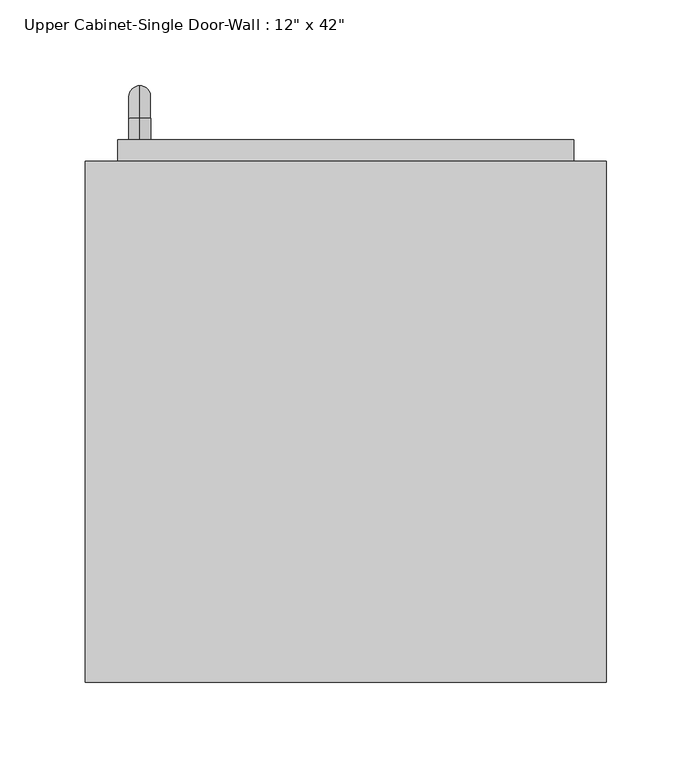
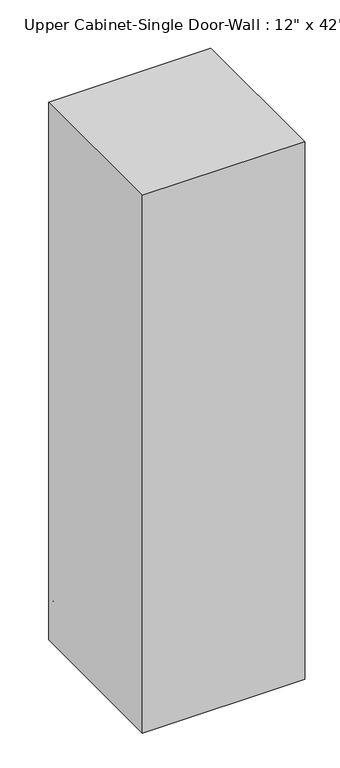
"""IFC4 building model written with IfcOpenShell, lengths in millimetres: furniture geometry."""

from ifc_helpers import new_model, si_unit, point, frame, origin, place, context, project, spatial, polyline, circle_curve, ellipse_curve, trimmed, outline, extrude, faceted_brep, source, transform, mapped, element, save
from ifc_brep_helpers import plane_surface, cylinder_surface, revolved_surface, advanced_brep


def furniture_d980f7c4(model_context):
    return source(origin(), model_context, "Body", "SolidModel", [
        faceted_brep([(-122.6288372, 61.9125, 2438.4), (-122.6288372, 61.9125, 1371.6), (182.1711628, 61.9125, 1371.6), (182.1711628, 61.9125, 2438.4), (-122.6288372, 366.7125, 2438.4), (182.1711628, 366.7125, 2438.4), (182.1711628, 366.7125, 1371.6), (-122.6288372, 366.7125, 1371.6), (-103.5788372, 366.7125, 2419.35), (-103.5788372, 366.7125, 1390.65), (163.1211628, 366.7125, 1390.65), (163.1211628, 366.7125, 2419.35), (163.1211628, 80.9625, 2419.35), (-103.5788372, 80.9625, 2419.35), (163.1211628, 80.9625, 1390.65), (-103.5788372, 80.9625, 1390.65)], [[[0, 1, 2, 3]], [[4, 5, 6, 7], [8, 9, 10, 11]], [[1, 0, 4, 7]], [[2, 1, 7, 6]], [[3, 2, 6, 5]], [[0, 3, 5, 4]], [[8, 11, 12, 13]], [[11, 10, 14, 12]], [[10, 9, 15, 14]], [[9, 8, 13, 15]], [[13, 12, 14, 15]]]),
        advanced_brep(
        [(-90.8788372, 379.4125, 1517.65), (-90.8788372, 379.4125, 1530.35), (-90.8788372, 392.1125, 1517.65), (-90.8788372, 392.1125, 1530.35), (-90.8788372, 411.1625, 1511.3), (-90.8788372, 398.4625, 1511.3), (-90.8788372, 398.4625, 1435.1), (-90.8788372, 411.1625, 1435.1), (-90.8788372, 392.1125, 1416.05), (-90.8788372, 392.1125, 1428.75), (-90.8788372, 379.4125, 1428.75), (-90.8788372, 379.4125, 1416.05)],
        [
            (0, 1, circle_curve(frame((-90.8788372, 379.4125, 1524.0), z_axis=(0.0, -1.0, 0.0), x_axis=(0.0, 0.0, 1.0)), 6.35)),
            (1, 0, circle_curve(frame((-90.8788372, 379.4125, 1524.0), z_axis=(0.0, -1.0, 0.0), x_axis=(0.0, 0.0, 1.0)), 6.35)),
            (0, 2),
            (2, 3, circle_curve(frame((-90.8788372, 392.1125, 1524.0), z_axis=(0.0, -1.0, 0.0), x_axis=(0.0, 0.0, 1.0)), 6.35)),
            (3, 1),
            (3, 2, circle_curve(frame((-90.8788372, 392.1125, 1524.0), z_axis=(0.0, -1.0, 0.0), x_axis=(0.0, 0.0, 1.0)), 6.35)),
            (4, 3, circle_curve(frame((-90.8788372, 392.1125, 1511.3), z_axis=(1.0, 0.0, 0.0), x_axis=(0.0, 0.0, 1.0)), 19.05)),
            (2, 5, circle_curve(frame((-90.8788372, 392.1125, 1511.3), z_axis=(-1.0, 0.0, 0.0), x_axis=(0.0, 0.0, 1.0)), 6.35)),
            (5, 4, circle_curve(frame((-90.8788372, 404.8125, 1511.3), z_axis=(0.0, 0.0, 1.0), x_axis=(0.0, 1.0, 0.0)), 6.35)),
            (4, 5, circle_curve(frame((-90.8788372, 404.8125, 1511.3), z_axis=(0.0, 0.0, 1.0), x_axis=(0.0, 1.0, 0.0)), 6.35)),
            (5, 6),
            (6, 7, circle_curve(frame((-90.8788372, 404.8125, 1435.1), z_axis=(0.0, 0.0, 1.0), x_axis=(0.0, 1.0, 0.0)), 6.35)),
            (7, 4),
            (7, 6, circle_curve(frame((-90.8788372, 404.8125, 1435.1), z_axis=(0.0, 0.0, 1.0), x_axis=(0.0, 1.0, 0.0)), 6.35)),
            (8, 7, circle_curve(frame((-90.8788372, 392.1125, 1435.1), z_axis=(1.0, 0.0, 0.0), x_axis=(0.0, 1.0, 0.0)), 19.05)),
            (6, 9, circle_curve(frame((-90.8788372, 392.1125, 1435.1), z_axis=(-1.0, 0.0, 0.0), x_axis=(0.0, 1.0, 0.0)), 6.35)),
            (9, 8, circle_curve(frame((-90.8788372, 392.1125, 1422.4), z_axis=(0.0, 1.0, 0.0), x_axis=(0.0, 0.0, -1.0)), 6.35)),
            (8, 9, circle_curve(frame((-90.8788372, 392.1125, 1422.4), z_axis=(0.0, 1.0, 0.0), x_axis=(0.0, 0.0, -1.0)), 6.35)),
            (10, 11, circle_curve(frame((-90.8788372, 379.4125, 1422.4), z_axis=(0.0, -1.0, 0.0), x_axis=(0.0, 0.0, -1.0)), 6.35)),
            (11, 10, circle_curve(frame((-90.8788372, 379.4125, 1422.4), z_axis=(0.0, -1.0, 0.0), x_axis=(0.0, 0.0, -1.0)), 6.35)),
            (9, 10),
            (11, 8),
        ],
        [
            plane_surface(frame((-97.2288372, 379.4125, 1524.0), z_axis=(0.0, -1.0, 0.0), x_axis=(0.0, 0.0, 1.0))),
            cylinder_surface(frame((-90.8788372, 379.4125, 1524.0), z_axis=(0.0, -1.0, 0.0), x_axis=(0.0, 0.0, 1.0)), 6.35),
            revolved_surface(trimmed(ellipse_curve(frame((-90.8788372, 392.1125, 1524.0), z_axis=(0.0, -1.0, 0.0), x_axis=(0.0, 0.0, 1.0)), 6.35, 6.35), [point((-90.8788372, 392.1125, 1517.65))], [point((-90.8788372, 392.1125, 1530.35))], True, "CARTESIAN"), (-90.8788372, 392.1125, 1511.3), (-1.0, 0.0, 0.0)),
            revolved_surface(trimmed(ellipse_curve(frame((-90.8788372, 392.1125, 1524.0), z_axis=(0.0, -1.0, 0.0), x_axis=(0.0, 0.0, 1.0)), 6.35, 6.35), [point((-90.8788372, 392.1125, 1530.35))], [point((-90.8788372, 392.1125, 1517.65))], True, "CARTESIAN"), (-90.8788372, 392.1125, 1511.3), (-1.0, 0.0, 0.0)),
            cylinder_surface(frame((-90.8788372, 404.8125, 1511.3), z_axis=(0.0, 0.0, 1.0), x_axis=(0.0, 1.0, 0.0)), 6.35),
            revolved_surface(trimmed(ellipse_curve(frame((-90.8788372, 404.8125, 1435.1), z_axis=(0.0, 0.0, 1.0), x_axis=(0.0, 1.0, 0.0)), 6.35, 6.35), [point((-90.8788372, 398.4625, 1435.1))], [point((-90.8788372, 411.1625, 1435.1))], True, "CARTESIAN"), (-90.8788372, 392.1125, 1435.1), (-1.0, 0.0, 0.0)),
            revolved_surface(trimmed(ellipse_curve(frame((-90.8788372, 404.8125, 1435.1), z_axis=(0.0, 0.0, 1.0), x_axis=(0.0, 1.0, 0.0)), 6.35, 6.35), [point((-90.8788372, 411.1625, 1435.1))], [point((-90.8788372, 398.4625, 1435.1))], True, "CARTESIAN"), (-90.8788372, 392.1125, 1435.1), (-1.0, 0.0, 0.0)),
            plane_surface(frame((-97.2288372, 379.4125, 1422.4), z_axis=(0.0, -1.0, 0.0), x_axis=(0.0, 0.0, -1.0))),
            cylinder_surface(frame((-90.8788372, 392.1125, 1422.4), z_axis=(0.0, 1.0, 0.0), x_axis=(0.0, 0.0, -1.0)), 6.35),
        ],
        [
            (0, [[1, 2]]),
            (1, [[-1, 3, 4, 5]]),
            (1, [[-2, -5, 6, -3]]),
            (2, [[7, -4, 8, 9]]),
            (3, [[-8, -6, -7, 10]]),
            (4, [[-9, 11, 12, 13]]),
            (4, [[-10, -13, 14, -11]]),
            (5, [[15, -12, 16, 17]]),
            (6, [[-16, -14, -15, 18]]),
            (7, [[19, 20]]),
            (8, [[-17, 21, -20, 22]]),
            (8, [[-18, -22, -19, -21]]),
        ],
    ),
        extrude(outline(polyline([(-103.5788372, 379.4125), (163.1211628, 379.4125), (163.1211628, 347.6625), (-103.5788372, 347.6625), (-103.5788372, 379.4125)])), frame((0.0, 0.0, 1390.65), z_axis=(0.0, 0.0, 1.0), x_axis=(1.0, 0.0, 0.0)), (0.0, 0.0, 1.0), 1028.7),
    ])


if __name__ == "__main__":
    model = new_model("IFC4")
    model_context = context("Model", 3, world=origin())
    ifc_project = project(units=[si_unit("LENGTHUNIT", "METRE", prefix="MILLI")], contexts=[model_context])
    site = spatial("IfcSite", under=ifc_project)
    building = spatial("IfcBuilding", under=site)
    placement = place(None, origin())
    furniture_shape = furniture_d980f7c4(model_context)
    element("IfcFurniture", 1, ObjectType="Upper Cabinet-Single Door-Wall : 12\" x 42\"", at=placement, inside=building, context=model_context, shape_type="MappedRepresentation", body=[
        mapped(furniture_shape, transform((0.0, 0.0, 0.0), x_axis=(1.0, 0.0, 0.0), y_axis=(0.0, 1.0, 0.0), z_axis=(0.0, 0.0, 1.0))),
    ])
    save(model, "model.ifc")

# Revit data of these elements
# Type "Upper Cabinet-Single Door-Wall : 12\" x 42\""
#   COBie.Type.CreatedBy = "doug.wood@us.ibm.com"
#   COBie.Type.CreatedOn = "2016-04-14T02:07:23"
#   COBie.Type.Name = "Casework_Upper Cabinet-Single Door-Wall_12\" x 42\""
#   COBie.Type.Category = "23-40 35 17 47 11 : Kitchen Casework"
#   COBie.Type.Description = "Upper Cabinet-Single Door-Wall_12\" x 42\""
#   COBie.Type.Manufacturer = ""
#   COBie.Type.ModelNumber = ""
#   Assembly Code = "C1030410"
#   COBie.Type.ReplacementCost = 0
#   Depth = 1' - 0"
#   Height = 3' - 6"
#   Top Of Cabinet = 8' - 0"
#   Width = 1' - 0"
#   COBie.Type = no
#   Cabinet Material = none
#   Door/Drawer Material = none
#   Handle Material = Cabinets - Handles
# Element 1 (IfcFurniture, "Upper Cabinet-Single Door-Wall : 12\" x 42\"")
#   Materials on its faces: "Cabinets", "Cabinets - Handles"
# Materials
#   "Cabinets - Handles": class "Metal", colour RGB 57 57 57, transparency 0
#   "Cabinets": class "Miscellaneous", colour RGB 249 249 249, transparency 0
